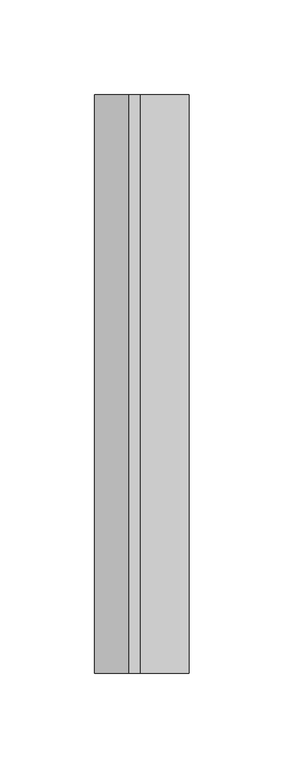
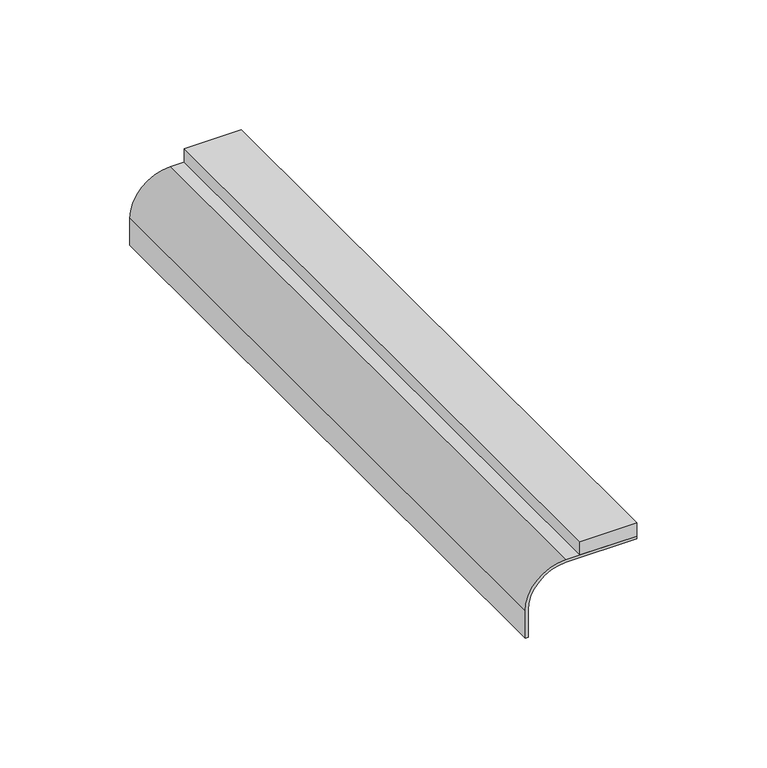
"""IFC4 building model written with IfcOpenShell, lengths in millimetres: proxy geometry, Generic Models 337:Generic Models 337:155472 : Generic Models 337:Generic Models 337:155472."""

from ifc_helpers import new_model, si_unit, point, frame, frame_2d, origin, place, context, project, spatial, polyline, circle_curve, trimmed, segment, composite_curve, outline, extrude, source, transform, mapped, element, save


def generic_models_e21651b4(model_context):
    return source(origin(), model_context, "Body", "SweptSolid", [
        extrude(outline(polyline([(8270.3053404, -3919.5173293), (8270.3053404, -3614.7173293), (8295.7053404, -3614.7173293), (8295.7053404, -3919.5173293), (8270.3053404, -3919.5173293)])), frame((0.0, 0.0, 2820.4732493), z_axis=(0.0, 0.0, 1.0), x_axis=(1.0, 0.0, 0.0)), (0.0, 0.0, 1.0), 6.35),
        extrude(outline(composite_curve([segment(polyline([(2820.4732493, 8295.7053404), (2820.4732493, 8263.9553404)]), True, "CONTINUOUS"), segment(trimmed(circle_curve(frame_2d((2802.5127371, 8263.9553404)), 17.9605122), [point((2820.4732493, 8263.9553404))], [point((2802.5127371, 8245.9948281))], False, "CARTESIAN"), True, "CONTINUOUS"), segment(polyline([(2802.5127371, 8245.9948281), (2789.8127371, 8245.9948281), (2789.8127371, 8247.2846719), (2802.5127371, 8247.2846719)]), True, "CONTINUOUS"), segment(trimmed(circle_curve(frame_2d((2802.5127371, 8263.9553404)), 16.6706685), [point((2802.5127371, 8247.2846719))], [point((2819.1834056, 8263.9553404))], True, "CARTESIAN"), True, "CONTINUOUS"), segment(polyline([(2819.1834056, 8263.9553404), (2819.1834056, 8295.7053404), (2820.4732493, 8295.7053404)]), True, "CONTINUOUS")], self_intersect=False)), frame((0.0, -3919.5173293, 0.0), z_axis=(0.0, 1.0, 0.0), x_axis=(0.0, 0.0, 1.0)), (0.0, 0.0, 1.0), 304.8),
    ])


if __name__ == "__main__":
    model = new_model("IFC4")
    model_context = context("Model", 3, world=origin())
    ifc_project = project(units=[si_unit("LENGTHUNIT", "METRE", prefix="MILLI")], contexts=[model_context])
    site = spatial("IfcSite", under=ifc_project)
    building = spatial("IfcBuilding", under=site)
    placement = place(None, origin())
    generic_models_shape = generic_models_e21651b4(model_context)
    element("IfcBuildingElementProxy", 1, Name="Generic Models 337:Generic Models 337:155472 : Generic Models 337:Generic Models 337:155472", ObjectType="Generic Models 337:Generic Models 337:155472 : Generic Models 337:Generic Models 337:155472", at=placement, inside=building, context=model_context, shape_type="MappedRepresentation", body=[
        mapped(generic_models_shape, transform((0.0, 0.0, 0.0), x_axis=(1.0, 0.0, 0.0), y_axis=(0.0, 1.0, 0.0), z_axis=(0.0, 0.0, 1.0))),
    ])
    save(model, "model.ifc")

# Revit data of these elements
# Type "Generic Models 337:Generic Models 337:155472 : Generic Models 337:Generic Models 337:155472"
#   NameOverride = "Generic Models 337:Generic Models 337:155472"
#   ObjectTypeOverride = "Generic Models 337:Generic Models 337"
#   Reference = "Generic Models 337"
#   Category = "Generic Models"
#   Tag = "155472"
# Element 1 (IfcBuildingElementProxy, "Generic Models 337:Generic Models 337:155472 : Generic Models 337:Generic Models 337:155472")
#   Materials on its faces: "_WEATHER STRIPPING 31845"
# Materials
#   "_WEATHER STRIPPING 31845": class "Unassigned", colour RGB 245 226 173, transparency 0
